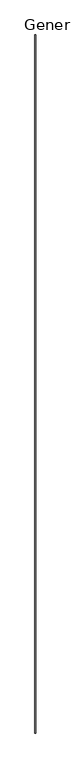
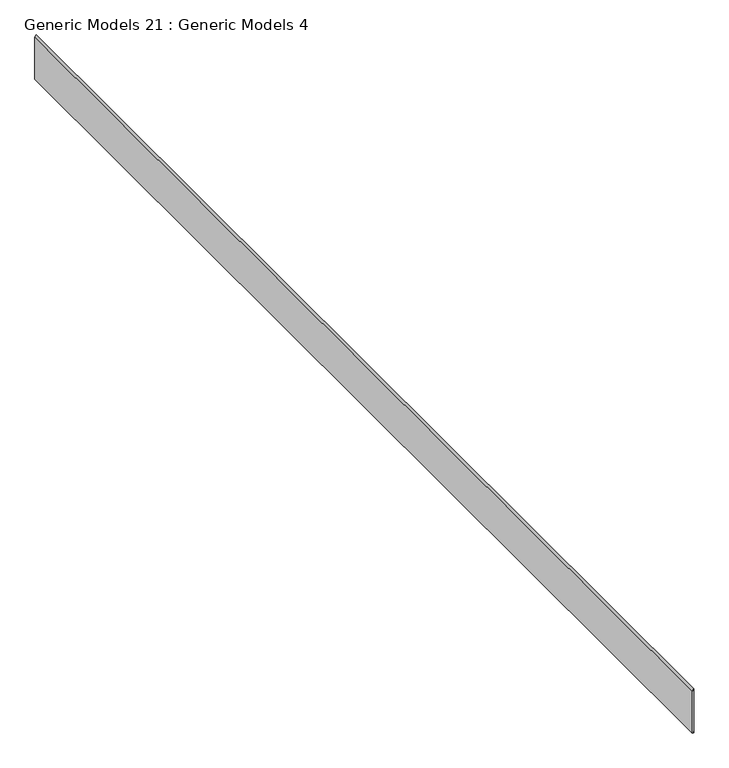
"""IFC4 building model written with IfcOpenShell, lengths in millimetres: proxy geometry, Generic Models 21 : Generic Models 4."""

import ifcopenshell
import ifcopenshell.guid

model = None  # the IFC model being written
_history = None  # IfcOwnerHistory: only IFC2X3 demands one
_inside = {}  # id of a spatial element -> (the spatial element, [elements in it])
_under = {}  # id of a project, library or spatial element -> (it, [spatial elements below it])
_declared = {}  # id of a project -> (the project, [libraries it declares])
_typed = {}  # id of a type object -> (the type object, [elements of that type])
_made_of = {}  # id of a material, layer set ... -> (it, [elements and type objects made of it])


def new_model(schema):
    """Start an empty IFC model of exactly this schema.

    Asked for "IFC4X3", IfcOpenShell would pick the latest addendum, in which some entities
    have other attributes; the version numbers below select the first issue.
    IFC2X3 requires an IfcOwnerHistory on every rooted entity: one is made here for all.
    """
    global model, _history
    if schema == "IFC4X3":
        model = ifcopenshell.file(schema_version=(4, 3, 0, 0))
    else:
        model = ifcopenshell.file(schema=schema)
    _inside.clear()
    _under.clear()
    _declared.clear()
    _typed.clear()
    _made_of.clear()
    _history = None
    if model.schema == "IFC2X3":
        org = make("IfcOrganization", Name="unknown")
        user = make(
            "IfcPersonAndOrganization",
            ThePerson=make("IfcPerson", FamilyName="unknown"),
            TheOrganization=org,
        )
        app = make(
            "IfcApplication",
            ApplicationDeveloper=org,
            Version="unknown",
            ApplicationFullName="unknown",
            ApplicationIdentifier="unknown",
        )
        _history = make(
            "IfcOwnerHistory",
            OwningUser=user,
            OwningApplication=app,
            ChangeAction="ADDED",
            CreationDate=0,
        )
    return model


def make(cls, **values):
    """One entity of the class cls with the attributes given. An attribute that is None is left unset."""
    return model.create_entity(
        cls, **{name: value for name, value in values.items() if value is not None}
    )


def rooted(cls, **values):
    """An entity with a GlobalId (a new one), such as an element, a storey or a relation."""
    return make(cls, GlobalId=ifcopenshell.guid.new(), OwnerHistory=_history, **values)


def si_unit(unit_type, name, prefix=None):
    """IfcSIUnit, for example si_unit("LENGTHUNIT", "METRE", prefix="MILLI")."""
    return make("IfcSIUnit", UnitType=unit_type, Prefix=prefix, Name=name)


def assignment(units):
    """IfcUnitAssignment: the units of a project."""
    return None if units is None else make("IfcUnitAssignment", Units=units)


def point(xyz):
    """IfcCartesianPoint."""
    return None if xyz is None else make("IfcCartesianPoint", Coordinates=xyz)


def direction(xyz):
    """IfcDirection."""
    return None if xyz is None else make("IfcDirection", DirectionRatios=xyz)


def frame(location, z_axis=None, x_axis=None):
    """IfcAxis2Placement3D, a coordinate frame: its origin and axes. An axis left out is left unset."""
    return make(
        "IfcAxis2Placement3D",
        Location=point(location),
        Axis=direction(z_axis),
        RefDirection=direction(x_axis),
    )


def origin():
    """The frame at (0, 0, 0) with its axes left unset."""
    return frame((0.0, 0.0, 0.0))


def place(relative_to, where):
    """IfcLocalPlacement: puts the frame where relative to a parent placement (None: the world)."""
    return make(
        "IfcLocalPlacement", PlacementRelTo=relative_to, RelativePlacement=where
    )


def context(
    kind, dimensions, precision=None, world=None, true_north=None, identifier=None
):
    """IfcGeometricRepresentationContext, for example the 3D "Model" context."""
    return make(
        "IfcGeometricRepresentationContext",
        ContextIdentifier=identifier,
        ContextType=kind,
        CoordinateSpaceDimension=dimensions,
        Precision=precision,
        WorldCoordinateSystem=world,
        TrueNorth=true_north,
    )


def project(units=None, contexts=None):
    """IfcProject with its units and contexts."""
    return rooted(
        "IfcProject",
        Name="project",
        RepresentationContexts=contexts,
        UnitsInContext=assignment(units),
    )


def spatial(cls, under=None, at=None, **own):
    """A site, building, storey or space (cls), placed at a placement, below another one or the project."""
    s = rooted(cls, ObjectPlacement=at, **own)
    if under is not None:
        _under.setdefault(under.id(), (under, []))[1].append(s)
    return s


def polyline(points):
    """IfcPolyline through the points."""
    return make("IfcPolyline", Points=[point(p) for p in points])


def outline(outer, holes=None, kind="AREA"):
    """IfcArbitraryClosedProfileDef: a profile drawn as a closed curve; with holes, ...WithVoids."""
    if holes is None:
        return make("IfcArbitraryClosedProfileDef", ProfileType=kind, OuterCurve=outer)
    return make(
        "IfcArbitraryProfileDefWithVoids",
        ProfileType=kind,
        OuterCurve=outer,
        InnerCurves=holes,
    )


def extrude(swept, where, along, depth):
    """IfcExtrudedAreaSolid: the profile swept, set in the frame where, extruded along a direction by depth."""
    return make(
        "IfcExtrudedAreaSolid",
        SweptArea=swept,
        Position=where,
        ExtrudedDirection=direction(along),
        Depth=depth,
    )


def shape(context_of_items, identifier, shape_type, items):
    """IfcShapeRepresentation: the items that make up one representation, for example the "Body"."""
    return make(
        "IfcShapeRepresentation",
        ContextOfItems=context_of_items,
        RepresentationIdentifier=identifier,
        RepresentationType=shape_type,
        Items=items,
    )


def source(mapping_origin, context_of_items, identifier, shape_type, items):
    """IfcRepresentationMap: a shape defined once, which mapped items show again and again."""
    return make(
        "IfcRepresentationMap",
        MappingOrigin=mapping_origin,
        MappedRepresentation=shape(context_of_items, identifier, shape_type, items),
    )


def transform(
    local_origin,
    x_axis=None,
    y_axis=None,
    z_axis=None,
    scale=None,
    scale2=None,
    scale3=None,
    uniform=True,
):
    """IfcCartesianTransformationOperator3D, or its non-uniform kind. x_axis, y_axis, z_axis: its Axis1, 2, 3."""
    if uniform:
        return make(
            "IfcCartesianTransformationOperator3D",
            Axis1=direction(x_axis),
            Axis2=direction(y_axis),
            LocalOrigin=point(local_origin),
            Scale=scale,
            Axis3=direction(z_axis),
        )
    return make(
        "IfcCartesianTransformationOperator3DnonUniform",
        Axis1=direction(x_axis),
        Axis2=direction(y_axis),
        LocalOrigin=point(local_origin),
        Scale=scale,
        Axis3=direction(z_axis),
        Scale2=scale2,
        Scale3=scale3,
    )


def mapped(mapping_source, mapping_target):
    """IfcMappedItem: shows the shape of a source again, moved by a transform."""
    return make(
        "IfcMappedItem", MappingSource=mapping_source, MappingTarget=mapping_target
    )


def made_of(thing, what):
    """Note that an element or type object is made of a material, layer set ...; save() writes the relation."""
    if what is not None:
        _made_of.setdefault(what.id(), (what, []))[1].append(thing)
    return thing


def element(
    cls,
    number,
    at=None,
    inside=None,
    cuts=None,
    type_object=None,
    material=None,
    context=None,
    identifier="Body",
    shape_type=None,
    held_by="IfcProductDefinitionShape",
    body=None,
    shapes=None,
    **own,
):
    """One element of the class cls, such as IfcWall. Its Tag is "e" and its number.

    at: its placement. inside: the storey or other place that contains it. cuts: it is an
    opening in that element (IfcRelVoidsElement). A single representation is given by context,
    identifier, shape_type and body (its items); several are given by shapes. held_by: the class
    of the entity that holds the representations. save() writes the other relations.
    """
    e = rooted(cls, Tag="e%d" % number, ObjectPlacement=at, **own)
    if body is not None:
        shapes = [shape(context, identifier, shape_type, body)]
    if shapes is not None:
        e.Representation = make(held_by, Representations=shapes)
    if inside is not None:
        _inside.setdefault(inside.id(), (inside, []))[1].append(e)
    if cuts is not None:
        rooted(
            "IfcRelVoidsElement", RelatingBuildingElement=cuts, RelatedOpeningElement=e
        )
    if type_object is not None:
        _typed.setdefault(type_object.id(), (type_object, []))[1].append(e)
    return made_of(e, material)


def aggregate(whole, parts):
    """IfcRelAggregates: a whole, such as a stair, and the parts it consists of."""
    return rooted("IfcRelAggregates", RelatingObject=whole, RelatedObjects=parts)


def save(model, path):
    """Write the relations noted so far, then the file.

    IfcRelAggregates (storeys below a building ...), IfcRelContainedInSpatialStructure (elements
    in a storey), IfcRelDefinesByType, IfcRelAssociatesMaterial and IfcRelDeclares: one each for
    every whole, place, type object, material and project.
    """
    for whole, parts in _under.values():
        aggregate(whole, parts)
    for where, things in _inside.values():
        rooted(
            "IfcRelContainedInSpatialStructure",
            RelatedElements=things,
            RelatingStructure=where,
        )
    for kind, things in _typed.values():
        rooted("IfcRelDefinesByType", RelatedObjects=things, RelatingType=kind)
    for what, things in _made_of.values():
        rooted("IfcRelAssociatesMaterial", RelatedObjects=things, RelatingMaterial=what)
    for by, libraries in _declared.values():
        rooted("IfcRelDeclares", RelatingContext=by, RelatedDefinitions=libraries)
    model.write(path)


def generic_models_21_generic_models_4_c3458904(model_context):
    return source(origin(), model_context, "Body", "SweptSolid", [
        extrude(outline(polyline([(127068.6707574, 8578.5852461), (126343.791, 8578.5852461), (126343.791, 8596.4563704), (126346.0008, 8596.4563704), (126346.0008, 8595.5975296), (126366.3153787, 8595.5975296), (126366.3153787, 8596.8675296), (126347.2708, 8596.8675296), (126347.2708, 8597.7263704), (127105.9455785, 8597.7263704), (127068.6707574, 8578.5852461)])), frame((0.0, -6864.9230338, 0.0), z_axis=(0.0, 1.0, 0.0), x_axis=(0.0, 0.0, 1.0)), (0.0, 0.0, 1.0), 18643.6),
    ])


if __name__ == "__main__":
    model = new_model("IFC4")
    model_context = context("Model", 3, world=origin())
    ifc_project = project(units=[si_unit("LENGTHUNIT", "METRE", prefix="MILLI")], contexts=[model_context])
    site = spatial("IfcSite", under=ifc_project)
    building = spatial("IfcBuilding", under=site)
    placement = place(None, origin())
    generic_models_21_generic_models_4_shape = generic_models_21_generic_models_4_c3458904(model_context)
    element("IfcBuildingElementProxy", 1, Name="Generic Models 21 : Generic Models 4", ObjectType="Generic Models 21 : Generic Models 4", at=placement, inside=building, context=model_context, shape_type="MappedRepresentation", body=[
        mapped(generic_models_21_generic_models_4_shape, transform((0.0, 0.0, 0.0), x_axis=(1.0, 0.0, 0.0), y_axis=(0.0, 1.0, 0.0), z_axis=(0.0, 0.0, 1.0))),
    ])
    save(model, "model.ifc")

# Revit data of these elements
# Element 1 (IfcBuildingElementProxy, "Generic Models 21 : Generic Models 4")
#   Materials on its faces: "_7/8\" SMOOTH TROWEL EXTERIOR STUCCO (COLOR PER OWNER)"
# Materials
#   "_7/8\" SMOOTH TROWEL EXTERIOR STUCCO (COLOR PER OWNER)": class "Generic", colour RGB 233 233 233, transparency 0, Cost = 0
